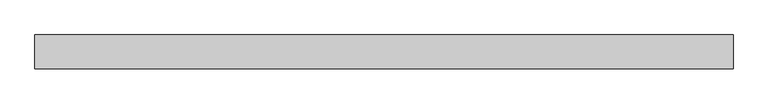
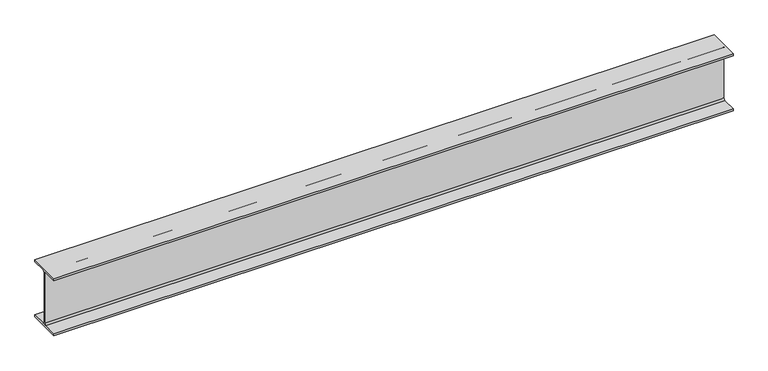
"""IFC4 building model written with IfcOpenShell, lengths in millimetres: beam geometry, Steel Beam_H-KSD3502 : H_SB_ASB_H-200x200x8x12."""

from ifc_helpers import new_model, si_unit, point, frame, frame_2d, origin, place, context, project, spatial, polyline, circle_curve, trimmed, segment, composite_curve, outline, extrude, source, transform, mapped, element, save


def beam_af1dc2e2(model_context):
    return source(origin(), model_context, "Body", "SweptSolid", [
        extrude(outline(composite_curve([segment(polyline([(-82.5, -141.5), (-11.9, -141.5)]), True, "CONTINUOUS"), segment(trimmed(circle_curve(frame_2d((-11.9, -132.6)), 8.9), [point((-11.9, -141.5))], [point((-3.0, -132.6))], True, "CARTESIAN"), True, "CONTINUOUS"), segment(polyline([(-3.0, -132.6), (-3.0, 132.6)]), True, "CONTINUOUS"), segment(trimmed(circle_curve(frame_2d((-11.9, 132.6)), 8.9), [point((-3.0, 132.6))], [point((-11.9, 141.5))], True, "CARTESIAN"), True, "CONTINUOUS"), segment(polyline([(-11.9, 141.5), (-82.5, 141.5), (-82.5, 151.7), (82.5, 151.7), (82.5, 141.5), (11.9, 141.5)]), True, "CONTINUOUS"), segment(trimmed(circle_curve(frame_2d((11.9, 132.6)), 8.9), [point((11.9, 141.5))], [point((3.0, 132.6))], True, "CARTESIAN"), True, "CONTINUOUS"), segment(polyline([(3.0, 132.6), (3.0, -132.6)]), True, "CONTINUOUS"), segment(trimmed(circle_curve(frame_2d((11.9, -132.6)), 8.9), [point((3.0, -132.6))], [point((11.9, -141.5))], True, "CARTESIAN"), True, "CONTINUOUS"), segment(polyline([(11.9, -141.5), (82.5, -141.5), (82.5, -151.7), (-82.5, -151.7), (-82.5, -141.5)]), True, "CONTINUOUS")], self_intersect=False)), frame((-1723.3906006, 0.0, 0.0), z_axis=(1.0, 0.0, 0.0), x_axis=(0.0, 1.0, 0.0)), (0.0, 0.0, 1.0), 3418.749313),
    ])


if __name__ == "__main__":
    model = new_model("IFC4")
    model_context = context("Model", 3, world=origin())
    ifc_project = project(units=[si_unit("LENGTHUNIT", "METRE", prefix="MILLI")], contexts=[model_context])
    site = spatial("IfcSite", under=ifc_project)
    building = spatial("IfcBuilding", under=site)
    placement = place(None, origin())
    beam_shape = beam_af1dc2e2(model_context)
    element("IfcBeam", 1, ObjectType="Steel Beam_H-KSD3502 : H_SB_ASB_H-200x200x8x12", at=placement, inside=building, context=model_context, shape_type="MappedRepresentation", body=[
        mapped(beam_shape, transform((0.0, 0.0, 0.0), x_axis=(1.0, 0.0, 0.0), y_axis=(0.0, 1.0, 0.0), z_axis=(0.0, 0.0, 1.0))),
    ])
    save(model, "model.ifc")

# Revit data of these elements
# Type "Steel Beam_H-KSD3502 : H_SB_ASB_H-200x200x8x12"
#   Width = 20.0 cm
#   Web Thickness = 0.8 cm
#   Web Fillet = 1.3 cm
#   Warping Constant = 141376.0 cm⁶
#   Torsional Moment of Inertia = 26.2485 cm⁴
#   Torsional Modulus = 1.0 cm³
#   Section Area = 63.53 cm²
#   Plastic Modulus weak axis = 244.0 cm³
#   Plastic Modulus strong axis = 525.0 cm³
#   Perimeter = 1.16 m²/m
#   Nominal Weight = 49.90 kgf/m
#   Moment of Inertia weak axis = 1600.00 cm⁴
#   Moment of Inertia strong axis = 4720.00 cm⁴
#   Height = 20.0 cm
#   Flange Thickness = 1.2 cm
#   Elastic Modulus weak axis = 160.0 cm³
#   Elastic Modulus strong axis = 472.0 cm³
#   Centroid Vertical = 10.0 cm
#   Centroid Horizontal = 10.0 cm
#   Length [instance default] = 1.5240 m
#   Structural Material [instance default] = Steel, 45-345
#   Assembly Code = ""
# Element 1 (IfcBeam, "Steel Beam_H-KSD3502 : H_SB_ASB_H-200x200x8x12")
#   Structural Material = none
# Materials
#   "Steel, 45-345": class "Metal", colour RGB 189 187 185, transparency 0, Description = "Steel 345 MPa", Cost = 0
